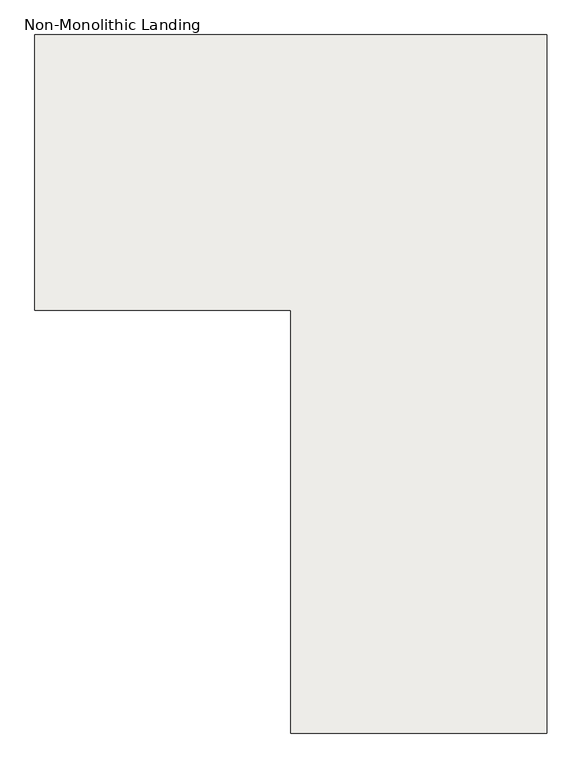
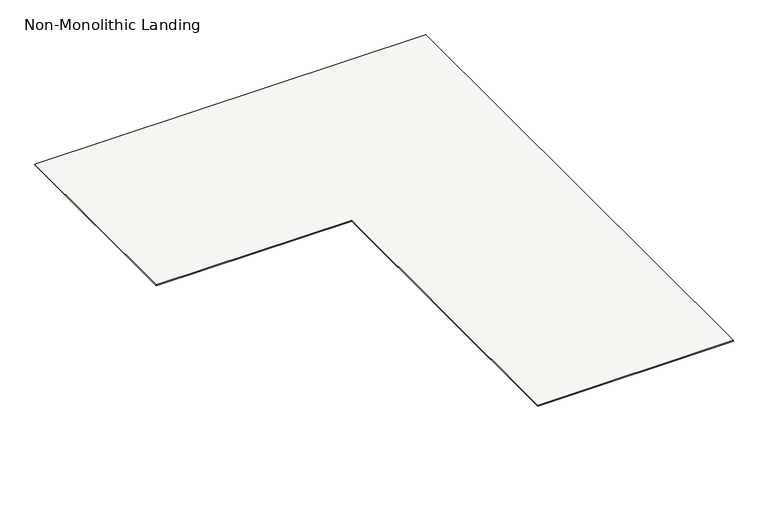
"""IFC4 building model written with IfcOpenShell, lengths in millimetres: slab geometry, Non-Monolithic Landing."""

from ifc_helpers import new_model, si_unit, origin, place, context, project, spatial, faceted_brep, source, transform, mapped, element, save


def non_monolithic_landing_788b4eaa(model_context):
    return source(origin(), model_context, "Body", "Brep", [
        faceted_brep([(-14425.0, 12030.4345331, 32000.0), (-13325.0, 12030.4345331, 32000.0), (-13325.0, 10214.4345331, 32000.0), (-12225.0, 10214.4345331, 32000.0), (-12225.0, 13214.4345331, 32000.0), (-14425.0, 13214.4345331, 32000.0), (-13325.0, 10214.4345331, 31994.0), (-13325.0, 12030.4345331, 31994.0), (-14424.15, 12030.4345331, 31994.0), (-14424.15, 13214.4345331, 31994.0), (-12225.0, 13214.4345331, 31994.0), (-12225.0, 10214.4345331, 31994.0)], [[[0, 1, 2, 3, 4, 5]], [[6, 7, 8, 9, 10, 11]], [[5, 4, 10, 9]], [[1, 0, 8, 7]], [[2, 1, 7, 6]], [[3, 2, 6, 11]], [[4, 3, 11, 10]], [[0, 5, 9, 8]]]),
    ])


if __name__ == "__main__":
    model = new_model("IFC4")
    model_context = context("Model", 3, world=origin())
    ifc_project = project(units=[si_unit("LENGTHUNIT", "METRE", prefix="MILLI")], contexts=[model_context])
    site = spatial("IfcSite", under=ifc_project)
    building = spatial("IfcBuilding", under=site)
    placement = place(None, origin())
    non_monolithic_landing_shape = non_monolithic_landing_788b4eaa(model_context)
    element("IfcSlab", 1, ObjectType="Non-Monolithic Landing", at=placement, inside=building, context=model_context, shape_type="MappedRepresentation", body=[
        mapped(non_monolithic_landing_shape, transform((0.0, 0.0, 0.0), x_axis=(1.0, 0.0, 0.0), y_axis=(0.0, 1.0, 0.0), z_axis=(0.0, 0.0, 1.0))),
    ])
    save(model, "model.ifc")

# Revit data of these elements
# Element 1 (IfcSlab, "Non-Monolithic Landing")
#   Materials on its faces: "Steel, Paint Finish, Dark Gray"
# Materials
#   "Steel, Paint Finish, Dark Gray": class "Metal", colour RGB 89 89 89, transparency 0, Description = "Steel, paint finish, dark gray, glossy", Cost = 0
